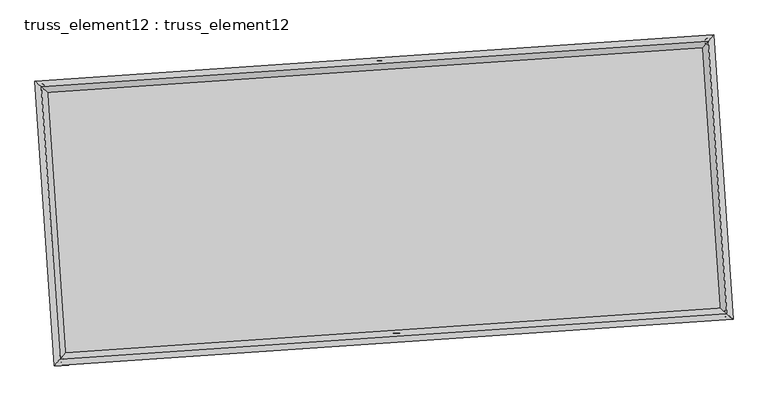
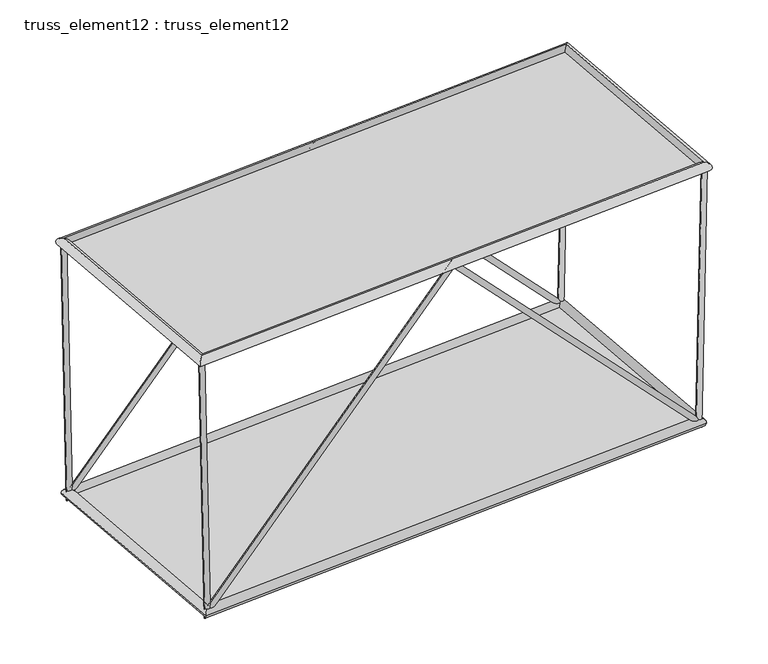
"""IFC4 building model written with IfcOpenShell, lengths in millimetres: plate geometry, truss_element12 : truss_element12."""

from ifc_helpers import new_model, si_unit, frame, origin, origin_with_axes, place, context, project, spatial, polyline, circle_curve, ellipse_curve, outline, extrude, source, transform, mapped, element, save
from ifc_brep_helpers import plane_surface, cylinder_surface, advanced_brep


def truss_element12_truss_element12_abe7b1e7(model_context):
    return source(origin(), model_context, "Body", "SolidModel", [
        advanced_brep(
        [(-3770.8878019, 2268.9998903, 4999.9319376), (-3869.9687215, 2255.6402044, 4997.8129357), (-3667.5052192, 2276.0491556, 121.4949725), (-3761.4816636, 2263.0375245, -121.4949725), (1064.3047665, 2598.6932913, 5070.9753827), (1064.7442266, 2592.1195217, 4926.7446167), (5794.9719015, 2921.2595003, 121.4870027), (5889.7890755, 2921.1209882, -121.4870027), (5899.4888428, 2928.3861132, 4999.9186849), (5999.4656666, 2928.5994181, 4997.7764407)],
        [
            (0, 1, circle_curve(frame((-3820.4282617, 2262.3200473, 4998.8724366), z_axis=(-0.021186964059823055, -0.0014446585400489402, 0.9997744873298331), x_axis=(-0.1335973438749746, 0.9910347078393886, -0.0013991308907449146)), 50.0)),
            (1, 0, circle_curve(frame((-3820.4282617, 2262.3200473, 4998.8724366), z_axis=(-0.021186964059823055, -0.0014446585400489402, 0.9997744873298331), x_axis=(-0.1335973438749746, 0.9910347078393886, -0.0013991308907449146)), 50.0)),
            (0, 2),
            (2, 3, ellipse_curve(frame((-3714.4934414, 2269.54334, 0.0), z_axis=(-0.9296544314303254, -0.06338960173189395, 0.36293855749180226), x_axis=(0.36209777260493814, 0.02469007065143342, 0.9318130732533052)), 130.6694735, 50.0)),
            (3, 1),
            (3, 2, ellipse_curve(frame((-3714.4934414, 2269.54334, 0.0), z_axis=(-0.9296544314303254, -0.06338960173189395, 0.36293855749180226), x_axis=(0.36209777260493814, 0.02469007065143342, 0.9318130732533052)), 130.6694735, 50.0)),
            (2, 4),
            (4, 5, ellipse_curve(frame((1064.5244965, 2595.4064065, 4998.8599997), z_axis=(-0.9976833942347468, -0.06802823810322978, 6.073553142189921e-05), x_axis=(-6.0594831251560616e-05, -4.131731200348947e-06, -0.9999999981555977)), 72.2724119, 50.0)),
            (5, 3),
            (5, 4, ellipse_curve(frame((1064.5244965, 2595.4064065, 4998.8599997), z_axis=(-0.9976833942347468, -0.06802823810322978, 6.073553142189921e-05), x_axis=(-6.0594831251560616e-05, -4.131731200348947e-06, -0.9999999981555977)), 72.2724119, 50.0)),
            (4, 6),
            (6, 7, ellipse_curve(frame((5842.3804885, 2921.1902443, 0.0), z_axis=(-0.929718590145964, -0.06339397647082363, -0.3627734098362472), x_axis=(-0.36193300753109015, -0.024678835947378536, 0.9318773809443935)), 130.6518852, 50.0)),
            (7, 5),
            (7, 6, ellipse_curve(frame((5842.3804885, 2921.1902443, 0.0), z_axis=(-0.929718590145964, -0.06339397647082363, -0.3627734098362472), x_axis=(-0.36193300753109015, -0.024678835947378536, 0.9318773809443935)), 130.6518852, 50.0)),
            (8, 9, circle_curve(frame((5949.4772547, 2928.4927656, 4998.8475628), z_axis=(0.021419353246380234, 0.001460504275286309, 0.9997695125546532), x_axis=(-0.0021638448984886293, 0.999996658509091, -0.0014144772560226867)), 50.0)),
            (9, 8, circle_curve(frame((5949.4772547, 2928.4927656, 4998.8475628), z_axis=(0.021419353246380234, 0.001460504275286309, 0.9997695125546532), x_axis=(-0.0021638448984886293, 0.999996658509091, -0.0014144772560226867)), 50.0)),
            (6, 8),
            (9, 7),
        ],
        [
            plane_surface(frame((-3820.4282617, 2312.3199951, 4998.9446858), z_axis=(-0.021186964059822382, -0.0014446585400488944, 0.9997744873298331), x_axis=(0.9997755310838168, -3.061480063770717e-05, 0.021186941940879226))),
            cylinder_surface(frame((-3820.4282617, 2262.3200473, 4998.8724366), z_axis=(-0.021186964059823055, -0.0014446585400489402, 0.9997744873298331), x_axis=(-0.1335973438749746, 0.9910347078393886, -0.0013991308907449146)), 50.0),
            cylinder_surface(frame((-3714.4934414, 2269.54334, 0.0), z_axis=(-0.6902679812639986, -0.047066749688142194, -0.7220213536423408), x_axis=(-0.02042071364567827, 0.9987517920300755, -0.045583465981802296)), 50.0),
            cylinder_surface(frame((1064.5244965, 2595.4064065, 4998.8599997), z_axis=(-0.6901804746474645, -0.0470607829446048, 0.7221053905933964), x_axis=(-0.11534567202188306, 0.9922792199619508, -0.045577687277029266)), 50.0),
            plane_surface(frame((5949.4772547, 2878.492819, 4998.9206047), z_axis=(0.02141935324638098, 0.0014605042752824204, 0.9997695125546532), x_axis=(0.999770579336333, -3.129023561676551e-05, -0.021419330391363928))),
            cylinder_surface(frame((5842.3804885, 2921.1902443, 0.0), z_axis=(-0.021419353246380234, -0.001460504275286309, -0.9997695125546532), x_axis=(-0.0021638448984886293, 0.999996658509091, -0.0014144772560226867)), 50.0),
        ],
        [
            (0, [[1, 2]]),
            (1, [[-1, 3, 4, 5]]),
            (1, [[-2, -5, 6, -3]]),
            (2, [[-4, 7, 8, 9]]),
            (2, [[-6, -9, 10, -7]]),
            (3, [[-8, 11, 12, 13]]),
            (3, [[-10, -13, 14, -11]]),
            (4, [[15, 16]]),
            (5, [[-12, 17, -16, 18]]),
            (5, [[-14, -18, -15, -17]]),
        ],
    ),
        advanced_brep(
        [(-3498.774849, -1721.733694, 4999.9319376), (-3597.8557686, -1735.0933799, 4997.8129357), (-3395.3922663, -1714.6844287, 121.4949725), (-3489.3687107, -1727.6960598, -121.4949725), (1336.4177194, -1392.040293, 5070.9753827), (1336.8571795, -1398.6140626, 4926.7446167), (6067.0848544, -1069.474084, 121.4870027), (6161.9020284, -1069.6125961, -121.4870027), (6171.6017958, -1062.3474711, 4999.9186849), (6271.5786195, -1062.1341662, 4997.7764407)],
        [
            (0, 1, circle_curve(frame((-3548.3153088, -1728.413537, 4998.8724366), z_axis=(-0.021186964059823104, -0.001444658540048999, 0.9997744873298331), x_axis=(-0.13359734387497507, 0.9910347078393886, -0.0013991308907448728)), 50.0)),
            (1, 0, circle_curve(frame((-3548.3153088, -1728.413537, 4998.8724366), z_axis=(-0.021186964059823104, -0.001444658540048999, 0.9997744873298331), x_axis=(-0.13359734387497507, 0.9910347078393886, -0.0013991308907448728)), 50.0)),
            (0, 2),
            (2, 3, ellipse_curve(frame((-3442.3804885, -1721.1902443, 0.0), z_axis=(-0.9296544314303253, -0.06338960173189416, 0.36293855749180204), x_axis=(0.3620977726049378, 0.02469007065143343, 0.9318130732533053)), 130.6694735, 50.0)),
            (3, 1),
            (3, 2, ellipse_curve(frame((-3442.3804885, -1721.1902443, 0.0), z_axis=(-0.9296544314303253, -0.06338960173189416, 0.36293855749180204), x_axis=(0.3620977726049378, 0.02469007065143343, 0.9318130732533053)), 130.6694735, 50.0)),
            (2, 4),
            (4, 5, ellipse_curve(frame((1336.6374494, -1395.3271778, 4998.8599997), z_axis=(-0.9976833942347471, -0.06802823810322975, 6.073553142173877e-05), x_axis=(-6.059483125109933e-05, -4.1317312005027025e-06, -0.9999999981555977)), 72.2724119, 50.0)),
            (5, 3),
            (5, 4, ellipse_curve(frame((1336.6374494, -1395.3271778, 4998.8599997), z_axis=(-0.9976833942347471, -0.06802823810322975, 6.073553142173877e-05), x_axis=(-6.059483125109933e-05, -4.1317312005027025e-06, -0.9999999981555977)), 72.2724119, 50.0)),
            (4, 6),
            (6, 7, ellipse_curve(frame((6114.4934414, -1069.54334, 0.0), z_axis=(-0.929718590145964, -0.06339397647082334, -0.3627734098362472), x_axis=(-0.36193300753109015, -0.024678835947378446, 0.9318773809443935)), 130.6518852, 50.0)),
            (7, 5),
            (7, 6, ellipse_curve(frame((6114.4934414, -1069.54334, 0.0), z_axis=(-0.929718590145964, -0.06339397647082334, -0.3627734098362472), x_axis=(-0.36193300753109015, -0.024678835947378446, 0.9318773809443935)), 130.6518852, 50.0)),
            (8, 9, circle_curve(frame((6221.5902076, -1062.2408187, 4998.8475628), z_axis=(0.021419353246380123, 0.0014605042752862665, 0.9997695125546532), x_axis=(-0.0021638448984882684, 0.999996658509091, -0.001414477256022652)), 50.0)),
            (9, 8, circle_curve(frame((6221.5902076, -1062.2408187, 4998.8475628), z_axis=(0.021419353246380123, 0.0014605042752862665, 0.9997695125546532), x_axis=(-0.0021638448984882684, 0.999996658509091, -0.001414477256022652)), 50.0)),
            (6, 8),
            (9, 7),
        ],
        [
            plane_surface(frame((-3548.3153088, -1678.4135892, 4998.9446858), z_axis=(-0.021186964059822382, -0.001444658540048914, 0.9997744873298331), x_axis=(0.9997755310838168, -3.061480063770717e-05, 0.021186941940879226))),
            cylinder_surface(frame((-3548.3153088, -1728.413537, 4998.8724366), z_axis=(-0.021186964059823104, -0.001444658540048999, 0.9997744873298331), x_axis=(-0.13359734387497507, 0.9910347078393886, -0.0013991308907448728)), 50.0),
            cylinder_surface(frame((-3442.3804885, -1721.1902443, 0.0), z_axis=(-0.6902679812639982, -0.04706674968814228, -0.722021353642341), x_axis=(-0.020420713645678303, 0.9987517920300755, -0.04558346598180237)), 50.0),
            cylinder_surface(frame((1336.6374494, -1395.3271778, 4998.8599997), z_axis=(-0.6901804746474646, -0.04706078294460461, 0.7221053905933964), x_axis=(-0.11534567202188295, 0.9922792199619508, -0.04557768727702941)), 50.0),
            plane_surface(frame((6221.5902076, -1112.2407653, 4998.9206047), z_axis=(0.021419353246380984, 0.0014605042752824403, 0.9997695125546533), x_axis=(0.999770579336333, -3.129023561676551e-05, -0.021419330391363928))),
            cylinder_surface(frame((6114.4934414, -1069.54334, 0.0), z_axis=(-0.021419353246380123, -0.0014605042752862665, -0.9997695125546532), x_axis=(-0.0021638448984882684, 0.999996658509091, -0.001414477256022652)), 50.0),
        ],
        [
            (0, [[1, 2]]),
            (1, [[-1, 3, 4, 5]]),
            (1, [[-2, -5, 6, -3]]),
            (2, [[-4, 7, 8, 9]]),
            (2, [[-6, -9, 10, -7]]),
            (3, [[-8, 11, 12, 13]]),
            (3, [[-10, -13, 14, -11]]),
            (4, [[15, 16]]),
            (5, [[-12, 17, -16, 18]]),
            (5, [[-14, -18, -15, -17]]),
        ],
    ),
        advanced_brep(
        [(-3548.3217778, -1728.4207068, 4908.8724369), (-3548.3088398, -1728.4063671, 5088.8724364), (-3820.4208794, 2262.313822, 5088.8724364), (-3820.4356441, 2262.3262727, 4908.8724369), (5949.4712419, 2928.4856269, 5088.8475625), (5949.4832676, 2928.4999043, 4908.847563), (6221.5832815, -1062.2345622, 5088.8475625), (6221.5971338, -1062.2470751, 4908.847563)],
        [
            (0, 1, ellipse_curve(frame((-3548.3153088, -1728.413537, 4998.8724366), z_axis=(-0.7535719234031808, 0.6573654662782376, 1.7961013785977973e-06), x_axis=(-0.6573654662758065, -0.7535719234053014, 1.7961013785979447e-06)), 127.2792206, 90.0)),
            (1, 2),
            (2, 3, ellipse_curve(frame((-3820.4282617, 2262.3200473, 4998.8724366), z_axis=(-0.6573654662758065, -0.7535719234053015, 1.796101378598083e-06), x_axis=(0.7535719234031809, -0.6573654662782374, -1.796101378597936e-06)), 127.2792206, 90.0)),
            (3, 0),
            (1, 0, ellipse_curve(frame((-3548.3153088, -1728.413537, 4998.8724366), z_axis=(-0.7535719234031808, 0.6573654662782376, 1.7961013785977973e-06), x_axis=(-0.6573654662758065, -0.7535719234053014, 1.7961013785979447e-06)), 127.2792206, 90.0)),
            (3, 2, ellipse_curve(frame((-3820.4282617, 2262.3200473, 4998.8724366), z_axis=(-0.6573654662758065, -0.7535719234053015, 1.796101378598083e-06), x_axis=(0.7535719234031809, -0.6573654662782374, -1.796101378597936e-06)), 127.2792206, 90.0)),
            (2, 4),
            (4, 5, ellipse_curve(frame((5949.4772547, 2928.4927656, 4998.8475628), z_axis=(-0.7535719234031808, 0.6573654662782376, 1.7961013785980747e-06), x_axis=(-0.6573654662758065, -0.7535719234053013, 1.796101378597944e-06)), 127.2792206, 90.0)),
            (5, 3),
            (5, 4, ellipse_curve(frame((5949.4772547, 2928.4927656, 4998.8475628), z_axis=(-0.7535719234031808, 0.6573654662782376, 1.7961013785980747e-06), x_axis=(-0.6573654662758065, -0.7535719234053013, 1.796101378597944e-06)), 127.2792206, 90.0)),
            (4, 6),
            (6, 7, ellipse_curve(frame((6221.5902076, -1062.2408187, 4998.8475628), z_axis=(0.6573654662758065, 0.7535719234053013, -1.7961013785978055e-06), x_axis=(-0.7535719234031807, 0.6573654662782378, 1.796101378597936e-06)), 127.2792206, 90.0)),
            (7, 5),
            (7, 6, ellipse_curve(frame((6221.5902076, -1062.2408187, 4998.8475628), z_axis=(0.6573654662758065, 0.7535719234053013, -1.7961013785978055e-06), x_axis=(-0.7535719234031807, 0.6573654662782378, 1.796101378597936e-06)), 127.2792206, 90.0)),
            (6, 1),
            (0, 7),
        ],
        [
            cylinder_surface(frame((-3548.3153088, -1728.413537, 4998.8724366), z_axis=(0.06802823822869959, -0.9976833960748769, 0.0), x_axis=(-0.9976833931072083, -0.06802823802634556, 7.713052989592242e-05)), 90.0),
            cylinder_surface(frame((-3820.4282617, 2262.3200473, 4998.8724366), z_axis=(-0.9976833960716583, -0.06802823822847938, 2.540070929010318e-06), x_axis=(-0.0680282378504271, 0.997683393312342, 7.459045897397833e-05)), 90.0),
            cylinder_surface(frame((5949.4772547, 2928.4927656, 4998.8475628), z_axis=(-0.06802823822869955, 0.997683396074877, 0.0), x_axis=(0.9976833934852606, 0.06802823805212346, 7.205038805203428e-05)), 90.0),
            cylinder_surface(frame((6221.5902076, -1062.2408187, 4998.8475628), z_axis=(0.9976833960716583, 0.06802823822847945, -2.5400709290101224e-06), x_axis=(0.06802823822847945, -0.997683393286564, 7.459045897397836e-05)), 90.0),
        ],
        [
            (0, [[1, 2, 3, 4]]),
            (0, [[5, -4, 6, -2]]),
            (1, [[-3, 7, 8, 9]]),
            (1, [[-6, -9, 10, -7]]),
            (2, [[-8, 11, 12, 13]]),
            (2, [[-10, -13, 14, -11]]),
            (3, [[-12, 15, -1, 16]]),
            (3, [[-14, -16, -5, -15]]),
        ],
    ),
        advanced_brep(
        [(-3358.7115243, -1625.2761972, 0.0), (-3526.0494527, -1817.1042913, 0.0), (-3810.4074885, 2353.2123043, 0.0), (-3618.5793943, 2185.8743758, 0.0), (5926.0494527, 3017.1042913, 0.0), (5758.7115243, 2825.2761972, 0.0), (6210.4074885, -1153.2123043, 0.0), (6018.5793943, -985.8743758, 0.0)],
        [
            (0, 1, ellipse_curve(frame((-3442.3804885, -1721.1902443, 0.0), z_axis=(-0.7535719234054581, 0.6573654662780808, 0.0), x_axis=(-0.6573654662780808, -0.7535719234054579, 0.0)), 127.2792206, 90.0)),
            (1, 2),
            (2, 3, ellipse_curve(frame((-3714.4934414, 2269.54334, 0.0), z_axis=(-0.6573654662780808, -0.753571923405458, 0.0), x_axis=(0.7535719234054581, -0.6573654662780807, 0.0)), 127.2792206, 90.0)),
            (3, 0),
            (1, 0, ellipse_curve(frame((-3442.3804885, -1721.1902443, 0.0), z_axis=(-0.7535719234054581, 0.6573654662780808, 0.0), x_axis=(-0.6573654662780808, -0.7535719234054579, 0.0)), 127.2792206, 90.0)),
            (3, 2, ellipse_curve(frame((-3714.4934414, 2269.54334, 0.0), z_axis=(-0.6573654662780808, -0.753571923405458, 0.0), x_axis=(0.7535719234054581, -0.6573654662780807, 0.0)), 127.2792206, 90.0)),
            (2, 4),
            (4, 5, ellipse_curve(frame((5842.3804885, 2921.1902443, 0.0), z_axis=(-0.7535719234054581, 0.6573654662780808, 0.0), x_axis=(-0.6573654662780806, -0.7535719234054581, 0.0)), 127.2792206, 90.0)),
            (5, 3),
            (5, 4, ellipse_curve(frame((5842.3804885, 2921.1902443, 0.0), z_axis=(-0.7535719234054581, 0.6573654662780808, 0.0), x_axis=(-0.6573654662780806, -0.7535719234054581, 0.0)), 127.2792206, 90.0)),
            (4, 6),
            (6, 7, ellipse_curve(frame((6114.4934414, -1069.54334, 0.0), z_axis=(0.6573654662780808, 0.753571923405458, 0.0), x_axis=(-0.753571923405458, 0.6573654662780808, 0.0)), 127.2792206, 90.0)),
            (7, 5),
            (7, 6, ellipse_curve(frame((6114.4934414, -1069.54334, 0.0), z_axis=(0.6573654662780808, 0.753571923405458, 0.0), x_axis=(-0.753571923405458, 0.6573654662780808, 0.0)), 127.2792206, 90.0)),
            (6, 1),
            (0, 7),
        ],
        [
            cylinder_surface(frame((-3442.3804885, -1721.1902443, 0.0), z_axis=(0.0680282382287018, -0.9976833960748765, 0.0), x_axis=(-0.9976833960748765, -0.0680282382287018, 0.0)), 90.0),
            cylinder_surface(frame((-3714.4934414, 2269.54334, 0.0), z_axis=(-0.9976833960748765, -0.06802823822870102, 0.0), x_axis=(-0.06802823822870102, 0.9976833960748765, 0.0)), 90.0),
            cylinder_surface(frame((5842.3804885, 2921.1902443, 0.0), z_axis=(-0.06802823822870162, 0.9976833960748765, 0.0), x_axis=(0.9976833960748765, 0.06802823822870162, 0.0)), 90.0),
            cylinder_surface(frame((6114.4934414, -1069.54334, 0.0), z_axis=(0.9976833960748767, 0.06802823822870084, 0.0), x_axis=(0.06802823822870084, -0.9976833960748767, 0.0)), 90.0),
        ],
        [
            (0, [[1, 2, 3, 4]]),
            (0, [[5, -4, 6, -2]]),
            (1, [[-3, 7, 8, 9]]),
            (1, [[-6, -9, 10, -7]]),
            (2, [[-8, 11, 12, 13]]),
            (2, [[-10, -13, 14, -11]]),
            (3, [[-12, 15, -1, 16]]),
            (3, [[-14, -16, -5, -15]]),
        ],
    ),
        extrude(outline(polyline([(-3442.3804885, -1721.1902443), (-3714.4934414, 2269.54334), (5842.3804885, 2921.1902443), (6114.4934414, -1069.54334), (-3442.3804885, -1721.1902443)])), origin_with_axes(), (0.0, 0.0, 1.0), 20.0),
        extrude(outline(polyline([(-2000.0, 4896.2955357), (2000.0, 4896.2955357), (2000.0, -4896.2955356), (-2000.0, -4896.2955356), (-2000.0, 4896.2955357)])), frame((1200.580973, 600.0396143, 4998.8599997), z_axis=(2.534186590725984e-06, 1.7279655027650736e-07, 0.9999999999967741), x_axis=(-0.06802823822870187, 0.9976833960748765, 0.0)), (0.0, 0.0, 1.0), 20.0),
    ])


if __name__ == "__main__":
    model = new_model("IFC4")
    model_context = context("Model", 3, world=origin())
    ifc_project = project(units=[si_unit("LENGTHUNIT", "METRE", prefix="MILLI")], contexts=[model_context])
    site = spatial("IfcSite", under=ifc_project)
    building = spatial("IfcBuilding", under=site)
    placement = place(None, origin())
    truss_element12_truss_element12_shape = truss_element12_truss_element12_abe7b1e7(model_context)
    element("IfcPlate", 1, ObjectType="truss_element12 : truss_element12", at=placement, inside=building, context=model_context, shape_type="MappedRepresentation", body=[
        mapped(truss_element12_truss_element12_shape, transform((0.0, 0.0, 0.0), x_axis=(1.0, 0.0, 0.0), y_axis=(0.0, 1.0, 0.0), z_axis=(0.0, 0.0, 1.0))),
    ])
    save(model, "model.ifc")

# Revit data of these elements
# Type "truss_element12 : truss_element12"
#   steellbar1 = 90 mm
#   steelbar2 = 50 mm
#   offset1 = 5000 mm
#   M = Default Roof
# Element 1 (IfcPlate, "truss_element12 : truss_element12")
#   Materials on its faces: "Default Roof"
# Materials
#   "Default Roof": class "Miscellaneous", colour RGB 0 127 0, transparency 0, Comments = "Rendering appearance not upgraded Rendering appearance not upgraded ", Cost = 0
